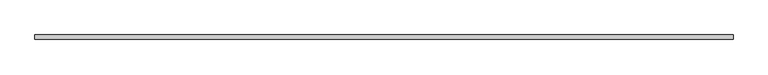
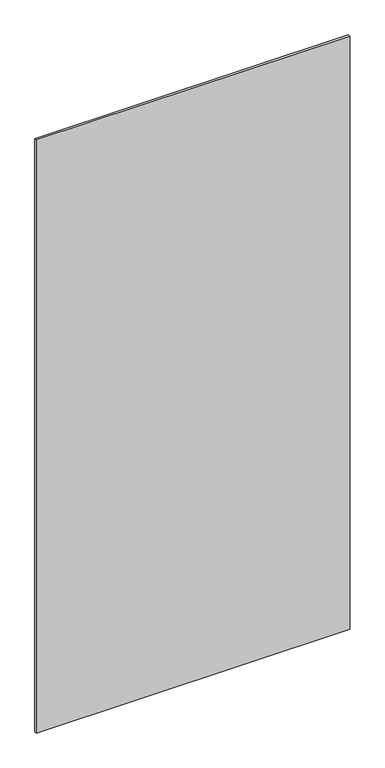
"""IFC4 building model written with IfcOpenShell, lengths in millimetres: proxy geometry, Panel:Panel:300402:Panel:300402 : Panel:Panel:300402:300124:Panel:300402:Panel:300402 : Panel:Panel:300402:300124 : Panel:Panel:300402:Panel:300402 : Panel:Panel:300402:300124:14 : Panel:Panel:300402:Panel:300402 : Panel:Panel:300402:300124:Panel:300402:Panel:300402 : Panel:Panel:300402:300124 : Panel:Panel:300402:Panel:300402 : Panel:Panel:300402:300124:300083."""

import ifcopenshell
import ifcopenshell.guid

model = None  # the IFC model being written
_history = None  # IfcOwnerHistory: only IFC2X3 demands one
_inside = {}  # id of a spatial element -> (the spatial element, [elements in it])
_under = {}  # id of a project, library or spatial element -> (it, [spatial elements below it])
_declared = {}  # id of a project -> (the project, [libraries it declares])
_typed = {}  # id of a type object -> (the type object, [elements of that type])
_made_of = {}  # id of a material, layer set ... -> (it, [elements and type objects made of it])


def new_model(schema):
    """Start an empty IFC model of exactly this schema.

    Asked for "IFC4X3", IfcOpenShell would pick the latest addendum, in which some entities
    have other attributes; the version numbers below select the first issue.
    IFC2X3 requires an IfcOwnerHistory on every rooted entity: one is made here for all.
    """
    global model, _history
    if schema == "IFC4X3":
        model = ifcopenshell.file(schema_version=(4, 3, 0, 0))
    else:
        model = ifcopenshell.file(schema=schema)
    _inside.clear()
    _under.clear()
    _declared.clear()
    _typed.clear()
    _made_of.clear()
    _history = None
    if model.schema == "IFC2X3":
        org = make("IfcOrganization", Name="unknown")
        user = make(
            "IfcPersonAndOrganization",
            ThePerson=make("IfcPerson", FamilyName="unknown"),
            TheOrganization=org,
        )
        app = make(
            "IfcApplication",
            ApplicationDeveloper=org,
            Version="unknown",
            ApplicationFullName="unknown",
            ApplicationIdentifier="unknown",
        )
        _history = make(
            "IfcOwnerHistory",
            OwningUser=user,
            OwningApplication=app,
            ChangeAction="ADDED",
            CreationDate=0,
        )
    return model


def make(cls, **values):
    """One entity of the class cls with the attributes given. An attribute that is None is left unset."""
    return model.create_entity(
        cls, **{name: value for name, value in values.items() if value is not None}
    )


def rooted(cls, **values):
    """An entity with a GlobalId (a new one), such as an element, a storey or a relation."""
    return make(cls, GlobalId=ifcopenshell.guid.new(), OwnerHistory=_history, **values)


def si_unit(unit_type, name, prefix=None):
    """IfcSIUnit, for example si_unit("LENGTHUNIT", "METRE", prefix="MILLI")."""
    return make("IfcSIUnit", UnitType=unit_type, Prefix=prefix, Name=name)


def assignment(units):
    """IfcUnitAssignment: the units of a project."""
    return None if units is None else make("IfcUnitAssignment", Units=units)


def point(xyz):
    """IfcCartesianPoint."""
    return None if xyz is None else make("IfcCartesianPoint", Coordinates=xyz)


def direction(xyz):
    """IfcDirection."""
    return None if xyz is None else make("IfcDirection", DirectionRatios=xyz)


def frame(location, z_axis=None, x_axis=None):
    """IfcAxis2Placement3D, a coordinate frame: its origin and axes. An axis left out is left unset."""
    return make(
        "IfcAxis2Placement3D",
        Location=point(location),
        Axis=direction(z_axis),
        RefDirection=direction(x_axis),
    )


def origin():
    """The frame at (0, 0, 0) with its axes left unset."""
    return frame((0.0, 0.0, 0.0))


def place(relative_to, where):
    """IfcLocalPlacement: puts the frame where relative to a parent placement (None: the world)."""
    return make(
        "IfcLocalPlacement", PlacementRelTo=relative_to, RelativePlacement=where
    )


def context(
    kind, dimensions, precision=None, world=None, true_north=None, identifier=None
):
    """IfcGeometricRepresentationContext, for example the 3D "Model" context."""
    return make(
        "IfcGeometricRepresentationContext",
        ContextIdentifier=identifier,
        ContextType=kind,
        CoordinateSpaceDimension=dimensions,
        Precision=precision,
        WorldCoordinateSystem=world,
        TrueNorth=true_north,
    )


def project(units=None, contexts=None):
    """IfcProject with its units and contexts."""
    return rooted(
        "IfcProject",
        Name="project",
        RepresentationContexts=contexts,
        UnitsInContext=assignment(units),
    )


def spatial(cls, under=None, at=None, **own):
    """A site, building, storey or space (cls), placed at a placement, below another one or the project."""
    s = rooted(cls, ObjectPlacement=at, **own)
    if under is not None:
        _under.setdefault(under.id(), (under, []))[1].append(s)
    return s


def polyline(points):
    """IfcPolyline through the points."""
    return make("IfcPolyline", Points=[point(p) for p in points])


def outline(outer, holes=None, kind="AREA"):
    """IfcArbitraryClosedProfileDef: a profile drawn as a closed curve; with holes, ...WithVoids."""
    if holes is None:
        return make("IfcArbitraryClosedProfileDef", ProfileType=kind, OuterCurve=outer)
    return make(
        "IfcArbitraryProfileDefWithVoids",
        ProfileType=kind,
        OuterCurve=outer,
        InnerCurves=holes,
    )


def extrude(swept, where, along, depth):
    """IfcExtrudedAreaSolid: the profile swept, set in the frame where, extruded along a direction by depth."""
    return make(
        "IfcExtrudedAreaSolid",
        SweptArea=swept,
        Position=where,
        ExtrudedDirection=direction(along),
        Depth=depth,
    )


def shape(context_of_items, identifier, shape_type, items):
    """IfcShapeRepresentation: the items that make up one representation, for example the "Body"."""
    return make(
        "IfcShapeRepresentation",
        ContextOfItems=context_of_items,
        RepresentationIdentifier=identifier,
        RepresentationType=shape_type,
        Items=items,
    )


def source(mapping_origin, context_of_items, identifier, shape_type, items):
    """IfcRepresentationMap: a shape defined once, which mapped items show again and again."""
    return make(
        "IfcRepresentationMap",
        MappingOrigin=mapping_origin,
        MappedRepresentation=shape(context_of_items, identifier, shape_type, items),
    )


def transform(
    local_origin,
    x_axis=None,
    y_axis=None,
    z_axis=None,
    scale=None,
    scale2=None,
    scale3=None,
    uniform=True,
):
    """IfcCartesianTransformationOperator3D, or its non-uniform kind. x_axis, y_axis, z_axis: its Axis1, 2, 3."""
    if uniform:
        return make(
            "IfcCartesianTransformationOperator3D",
            Axis1=direction(x_axis),
            Axis2=direction(y_axis),
            LocalOrigin=point(local_origin),
            Scale=scale,
            Axis3=direction(z_axis),
        )
    return make(
        "IfcCartesianTransformationOperator3DnonUniform",
        Axis1=direction(x_axis),
        Axis2=direction(y_axis),
        LocalOrigin=point(local_origin),
        Scale=scale,
        Axis3=direction(z_axis),
        Scale2=scale2,
        Scale3=scale3,
    )


def mapped(mapping_source, mapping_target):
    """IfcMappedItem: shows the shape of a source again, moved by a transform."""
    return make(
        "IfcMappedItem", MappingSource=mapping_source, MappingTarget=mapping_target
    )


def made_of(thing, what):
    """Note that an element or type object is made of a material, layer set ...; save() writes the relation."""
    if what is not None:
        _made_of.setdefault(what.id(), (what, []))[1].append(thing)
    return thing


def element(
    cls,
    number,
    at=None,
    inside=None,
    cuts=None,
    type_object=None,
    material=None,
    context=None,
    identifier="Body",
    shape_type=None,
    held_by="IfcProductDefinitionShape",
    body=None,
    shapes=None,
    **own,
):
    """One element of the class cls, such as IfcWall. Its Tag is "e" and its number.

    at: its placement. inside: the storey or other place that contains it. cuts: it is an
    opening in that element (IfcRelVoidsElement). A single representation is given by context,
    identifier, shape_type and body (its items); several are given by shapes. held_by: the class
    of the entity that holds the representations. save() writes the other relations.
    """
    e = rooted(cls, Tag="e%d" % number, ObjectPlacement=at, **own)
    if body is not None:
        shapes = [shape(context, identifier, shape_type, body)]
    if shapes is not None:
        e.Representation = make(held_by, Representations=shapes)
    if inside is not None:
        _inside.setdefault(inside.id(), (inside, []))[1].append(e)
    if cuts is not None:
        rooted(
            "IfcRelVoidsElement", RelatingBuildingElement=cuts, RelatedOpeningElement=e
        )
    if type_object is not None:
        _typed.setdefault(type_object.id(), (type_object, []))[1].append(e)
    return made_of(e, material)


def aggregate(whole, parts):
    """IfcRelAggregates: a whole, such as a stair, and the parts it consists of."""
    return rooted("IfcRelAggregates", RelatingObject=whole, RelatedObjects=parts)


def save(model, path):
    """Write the relations noted so far, then the file.

    IfcRelAggregates (storeys below a building ...), IfcRelContainedInSpatialStructure (elements
    in a storey), IfcRelDefinesByType, IfcRelAssociatesMaterial and IfcRelDeclares: one each for
    every whole, place, type object, material and project.
    """
    for whole, parts in _under.values():
        aggregate(whole, parts)
    for where, things in _inside.values():
        rooted(
            "IfcRelContainedInSpatialStructure",
            RelatedElements=things,
            RelatingStructure=where,
        )
    for kind, things in _typed.values():
        rooted("IfcRelDefinesByType", RelatedObjects=things, RelatingType=kind)
    for what, things in _made_of.values():
        rooted("IfcRelAssociatesMaterial", RelatedObjects=things, RelatingMaterial=what)
    for by, libraries in _declared.values():
        rooted("IfcRelDeclares", RelatingContext=by, RelatedDefinitions=libraries)
    model.write(path)


def generic_models_16cc9648(model_context):
    return source(origin(), model_context, "Body", "SweptSolid", [
        extrude(outline(polyline([(560648.2367239, -579076.8913841), (561867.4367239, -579076.8913841), (561867.4367239, -579084.8288841), (560648.2367239, -579084.8288841), (560648.2367239, -579076.8913841)])), frame((0.0, 0.0, 3695.7), z_axis=(0.0, 0.0, 1.0), x_axis=(1.0, 0.0, 0.0)), (0.0, 0.0, 1.0), 2438.4),
    ])


if __name__ == "__main__":
    model = new_model("IFC4")
    model_context = context("Model", 3, world=origin())
    ifc_project = project(units=[si_unit("LENGTHUNIT", "METRE", prefix="MILLI")], contexts=[model_context])
    site = spatial("IfcSite", under=ifc_project)
    building = spatial("IfcBuilding", under=site)
    placement = place(None, origin())
    generic_models_shape = generic_models_16cc9648(model_context)
    element("IfcBuildingElementProxy", 1, Name="Panel:Panel:300402:Panel:300402 : Panel:Panel:300402:300124:Panel:300402:Panel:300402 : Panel:Panel:300402:300124 : Panel:Panel:300402:Panel:300402 : Panel:Panel:300402:300124:14 : Panel:Panel:300402:Panel:300402 : Panel:Panel:300402:300124:Panel:300402:Panel:300402 : Panel:Panel:300402:300124 : Panel:Panel:300402:Panel:300402 : Panel:Panel:300402:300124:300083", ObjectType="Panel:Panel:300402:Panel:300402 : Panel:Panel:300402:300124:Panel:300402:Panel:300402 : Panel:Panel:300402:300124 : Panel:Panel:300402:Panel:300402 : Panel:Panel:300402:300124:14 : Panel:Panel:300402:Panel:300402 : Panel:Panel:300402:300124:Panel:300402:Panel:300402 : Panel:Panel:300402:300124 : Panel:Panel:300402:Panel:300402 : Panel:Panel:300402:300124:300083", at=placement, inside=building, context=model_context, shape_type="MappedRepresentation", body=[
        mapped(generic_models_shape, transform((0.0, 0.0, 0.0), x_axis=(1.0, 0.0, 0.0), y_axis=(0.0, 1.0, 0.0), z_axis=(0.0, 0.0, 1.0))),
    ])
    save(model, "model.ifc")

# Revit data of these elements
# Type "Panel:Panel:300402:Panel:300402 : Panel:Panel:300402:300124:Panel:300402:Panel:300402 : Panel:Panel:300402:300124 : Panel:Panel:300402:Panel:300402 : Panel:Panel:300402:300124:14 : Panel:Panel:300402:Panel:300402 : Panel:Panel:300402:300124:Panel:300402:Panel:300402 : Panel:Panel:300402:300124 : Panel:Panel:300402:Panel:300402 : Panel:Panel:300402:300124:300083"
#   NameOverride = "Panel:Panel:300402:Panel:300402 : Panel:Panel:300402:300124:Panel:300402:Panel:300402 : Panel:Panel:300402:300124 : Panel:Panel:300402:Panel:300402 : Panel:Panel:300402:300124:300083"
#   ObjectTypeOverride = "Panel:300402:Panel:300402 : Panel:Panel:300402:300124 : Panel:Panel:300402:Panel:300402 : Panel:Panel:300402:300124"
#   Reference = "Panel"
#   Tag = "300083"
# Element 1 (IfcBuildingElementProxy, "Panel:Panel:300402:Panel:300402 : Panel:Panel:300402:300124:Panel:300402:Panel:300402 : Panel:Panel:300402:300124 : Panel:Panel:300402:Panel:300402 : Panel:Panel:300402:300124:14 : Panel:Panel:300402:Panel:300402 : Panel:Panel:300402:300124:Panel:300402:Panel:300402 : Panel:Panel:300402:300124 : Panel:Panel:300402:Panel:300402 : Panel:Panel:300402:300124:300083")
#   Materials on its faces: "5/16\" THICK STONEWOOD RESIN PANELS - EXPOSED FASTENERS"
# Materials
#   "5/16\" THICK STONEWOOD RESIN PANELS - EXPOSED FASTENERS": class "Unassigned", colour RGB 64 64 64, transparency 0, Keynote = "M07420000.01", Cost = 0
